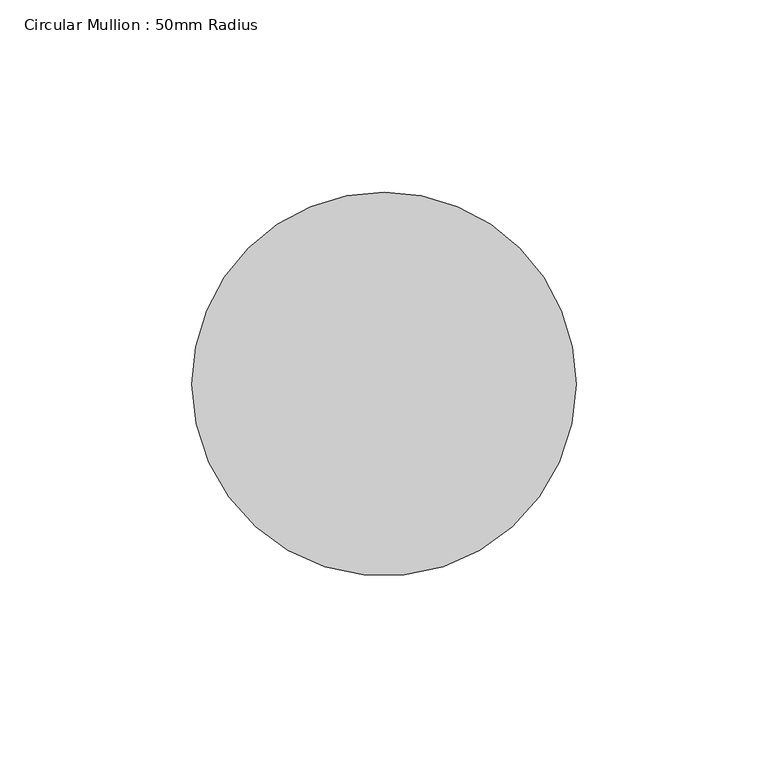
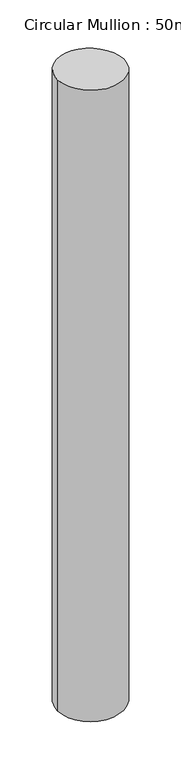
"""IFC4 building model written with IfcOpenShell, lengths in millimetres: member geometry, Circular Mullion : 50mm Radius."""

from ifc_helpers import new_model, si_unit, frame, origin, place, context, project, spatial, ellipse_curve, source, transform, mapped, element, save
from ifc_brep_helpers import plane_surface, cylinder_surface, advanced_brep


def circular_mullion_50mm_radius_9cb17007(model_context):
    return source(origin(), model_context, "Body", "AdvancedBrep", [
        advanced_brep(
        [(-100.0, 0.0, 2.2705131), (0.0, 0.0, 0.0), (0.0, 0.0, -1001.967576), (-100.0, 0.0, -1004.2466892)],
        [
            (0, 1, ellipse_curve(frame((-50.0, 0.0, 1.1352565), z_axis=(-0.02269369286962266, -0.02218671989148109, -0.9994962459981509), x_axis=(-0.7146884919686058, -0.6987224808262837, 0.03173726887436502)), 50.0252004, 50.0)),
            (1, 2),
            (2, 3, ellipse_curve(frame((-50.0, 0.0, -1003.1071326), z_axis=(-0.02277956339408985, -0.022270672084023665, 0.99949242551232), x_axis=(0.7146857601351735, 0.6987198100215204, 0.03185735933029571)), 50.0253916, 50.0)),
            (3, 0),
            (1, 0, ellipse_curve(frame((-50.0, 0.0, 1.1352565), z_axis=(-0.02269369286962266, -0.02218671989148109, -0.9994962459981509), x_axis=(-0.7146884919686058, -0.6987224808262837, 0.03173726887436502)), 50.0252004, 50.0)),
            (3, 2, ellipse_curve(frame((-50.0, 0.0, -1003.1071326), z_axis=(-0.02277956339408985, -0.022270672084023665, 0.99949242551232), x_axis=(0.7146857601351735, 0.6987198100215204, 0.03185735933029571)), 50.0253916, 50.0)),
        ],
        [
            cylinder_surface(frame((-50.0, 0.0, 0.0), z_axis=(0.0, 0.0, 1.0), x_axis=(1.0, 0.0, 0.0)), 50.0),
            plane_surface(frame((-213.077951, 217.9468439, 0.0), z_axis=(0.022693692869622663, 0.022186719891481094, 0.9994962459981511), x_axis=(0.7146884919686055, 0.6987224808262841, -0.03173726887436607))),
            plane_surface(frame((-213.077951, 217.9468439, -1001.967576), z_axis=(0.02277956339408985, 0.022270672084023665, -0.99949242551232), x_axis=(0.7146857601351736, 0.6987198100215205, 0.03185735933029399))),
        ],
        [
            (0, [[1, 2, 3, 4]]),
            (0, [[5, -4, 6, -2]]),
            (1, [[-1, -5]]),
            (2, [[-6, -3]]),
        ],
    ),
    ])


if __name__ == "__main__":
    model = new_model("IFC4")
    model_context = context("Model", 3, world=origin())
    ifc_project = project(units=[si_unit("LENGTHUNIT", "METRE", prefix="MILLI")], contexts=[model_context])
    site = spatial("IfcSite", under=ifc_project)
    building = spatial("IfcBuilding", under=site)
    placement = place(None, origin())
    circular_mullion_50mm_radius_shape = circular_mullion_50mm_radius_9cb17007(model_context)
    element("IfcMember", 1, ObjectType="Circular Mullion : 50mm Radius", at=placement, inside=building, context=model_context, shape_type="MappedRepresentation", body=[
        mapped(circular_mullion_50mm_radius_shape, transform((0.0, 0.0, 0.0), x_axis=(1.0, 0.0, 0.0), y_axis=(0.0, 1.0, 0.0), z_axis=(0.0, 0.0, 1.0))),
    ])
    save(model, "model.ifc")

# Revit data of these elements
# Type "Circular Mullion : 50mm Radius"
#   built-in parameter 1007350 = 0.164042 (stored number, unit not read)
# Element 1 (IfcMember, "Circular Mullion : 50mm Radius")
#   Materials on its faces: "Aluminium"
# Materials
#   "Aluminium": class "Metal", colour RGB 247 247 247, transparency 0, Description = "Aluminium 6061", Cost = 0
